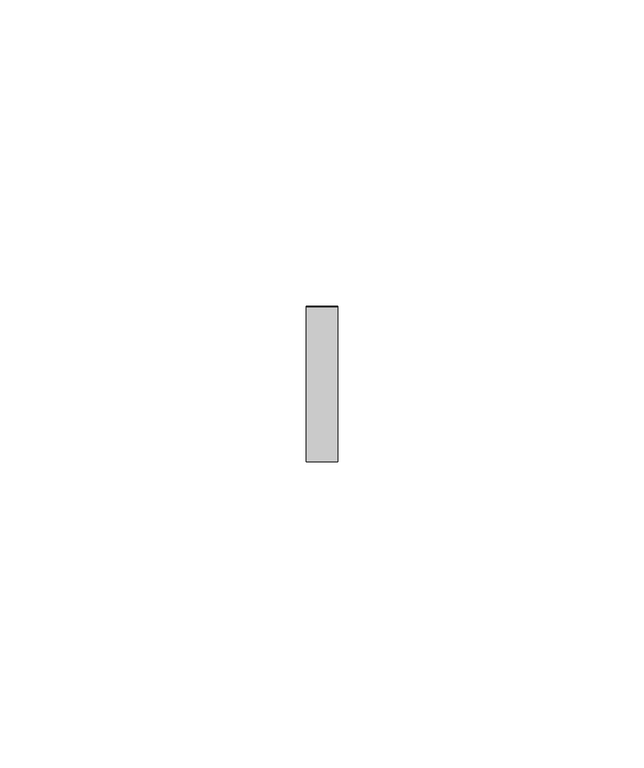
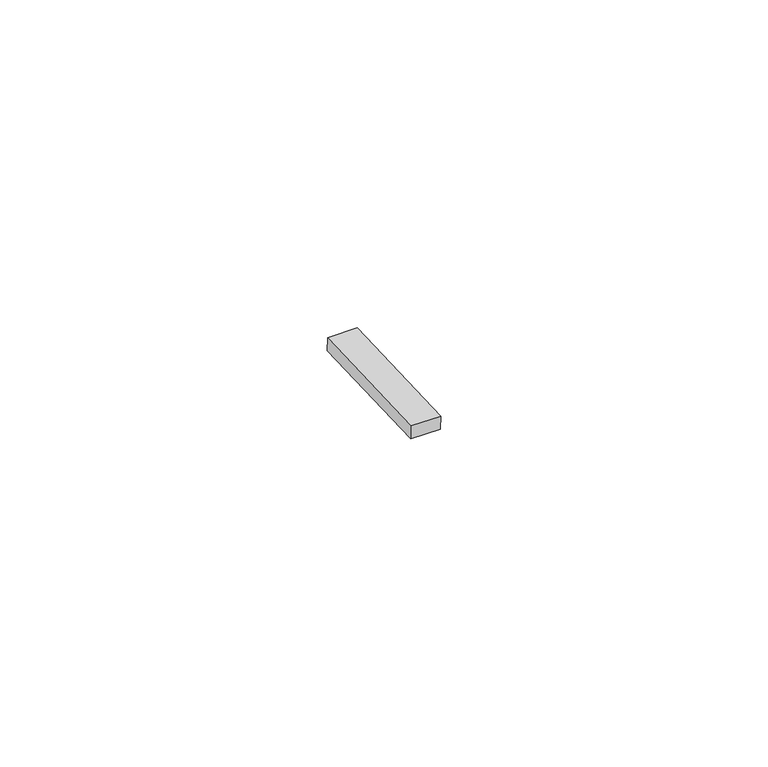
"""IFC4 building model written with IfcOpenShell, lengths in millimetres: proxy geometry, Inner panel:Inner panel:1:Inner panel:1 : Inner panel:Inner panel:300324:2:Inner panel:1:Inner panel:1 : Inner panel:Inner panel:300324:2 : Inner panel:Inner panel:1:Inner panel:1 : Inner panel:Inner panel:300324:300043:125 : Inner panel:Inner panel:1:Inner panel:1 : Inner panel:Inner panel:300324:2:Inner panel:1:Inner panel:1 : Inner panel:Inner panel:300324:2 : Inner panel:Inner panel:1:Inner panel:1 : Inner panel:Inner panel:300324:300043:308120."""

from ifc_helpers import new_model, si_unit, frame, origin, place, context, project, spatial, polyline, outline, extrude, source, transform, mapped, element, save


def generic_models_ade7059a(model_context):
    return source(origin(), model_context, "Body", "SweptSolid", [
        extrude(outline(polyline([(0.0, -25.4), (0.0, 0.0), (5.2138089, 0.0), (5.2138089, -25.4), (0.0, -25.4)])), frame((591904.595117, -578253.2828061, 3981.0403755), z_axis=(0.0, -0.041630544712223896, 0.9991330730923502), x_axis=(-1.0, 0.0, 0.0)), (0.0, 0.0, 1.0), 2.4763745),
    ])


if __name__ == "__main__":
    model = new_model("IFC4")
    model_context = context("Model", 3, world=origin())
    ifc_project = project(units=[si_unit("LENGTHUNIT", "METRE", prefix="MILLI")], contexts=[model_context])
    site = spatial("IfcSite", under=ifc_project)
    building = spatial("IfcBuilding", under=site)
    placement = place(None, origin())
    generic_models_shape = generic_models_ade7059a(model_context)
    element("IfcBuildingElementProxy", 1, Name="Inner panel:Inner panel:1:Inner panel:1 : Inner panel:Inner panel:300324:2:Inner panel:1:Inner panel:1 : Inner panel:Inner panel:300324:2 : Inner panel:Inner panel:1:Inner panel:1 : Inner panel:Inner panel:300324:300043:125 : Inner panel:Inner panel:1:Inner panel:1 : Inner panel:Inner panel:300324:2:Inner panel:1:Inner panel:1 : Inner panel:Inner panel:300324:2 : Inner panel:Inner panel:1:Inner panel:1 : Inner panel:Inner panel:300324:300043:308120", ObjectType="Inner panel:Inner panel:1:Inner panel:1 : Inner panel:Inner panel:300324:2:Inner panel:1:Inner panel:1 : Inner panel:Inner panel:300324:2 : Inner panel:Inner panel:1:Inner panel:1 : Inner panel:Inner panel:300324:300043:125 : Inner panel:Inner panel:1:Inner panel:1 : Inner panel:Inner panel:300324:2:Inner panel:1:Inner panel:1 : Inner panel:Inner panel:300324:2 : Inner panel:Inner panel:1:Inner panel:1 : Inner panel:Inner panel:300324:300043:308120", at=placement, inside=building, context=model_context, shape_type="MappedRepresentation", body=[
        mapped(generic_models_shape, transform((0.0, 0.0, 0.0), x_axis=(1.0, 0.0, 0.0), y_axis=(0.0, 1.0, 0.0), z_axis=(0.0, 0.0, 1.0))),
    ])
    save(model, "model.ifc")

# Revit data of these elements
# Type "Inner panel:Inner panel:1:Inner panel:1 : Inner panel:Inner panel:300324:2:Inner panel:1:Inner panel:1 : Inner panel:Inner panel:300324:2 : Inner panel:Inner panel:1:Inner panel:1 : Inner panel:Inner panel:300324:300043:125 : Inner panel:Inner panel:1:Inner panel:1 : Inner panel:Inner panel:300324:2:Inner panel:1:Inner panel:1 : Inner panel:Inner panel:300324:2 : Inner panel:Inner panel:1:Inner panel:1 : Inner panel:Inner panel:300324:300043:308120"
#   NameOverride = "Inner panel:Inner panel:1:Inner panel:1 : Inner panel:Inner panel:300324:2:Inner panel:1:Inner panel:1 : Inner panel:Inner panel:300324:2 : Inner panel:Inner panel:1:Inner panel:1 : Inner panel:Inner panel:300324:300043:308120"
#   ObjectTypeOverride = "Inner panel:1:Inner panel:1 : Inner panel:Inner panel:300324:2 : Inner panel:Inner panel:1:Inner panel:1 : Inner panel:Inner panel:300324:300043"
#   Reference = "Inner panel"
#   Tag = "308120"
# Element 1 (IfcBuildingElementProxy, "Inner panel:Inner panel:1:Inner panel:1 : Inner panel:Inner panel:300324:2:Inner panel:1:Inner panel:1 : Inner panel:Inner panel:300324:2 : Inner panel:Inner panel:1:Inner panel:1 : Inner panel:Inner panel:300324:300043:125 : Inner panel:Inner panel:1:Inner panel:1 : Inner panel:Inner panel:300324:2:Inner panel:1:Inner panel:1 : Inner panel:Inner panel:300324:2 : Inner panel:Inner panel:1:Inner panel:1 : Inner panel:Inner panel:300324:300043:308120")
#   Materials on its faces: "AT CLIP - 1\" WIDE NON ABSORBENT, WEATHER-RESISTANT NEOPRENE/EPDM/SBR FOAM"
# Materials
#   "AT CLIP - 1\" WIDE NON ABSORBENT, WEATHER-RESISTANT NEOPRENE/EPDM/SBR FOAM": class "Generic", colour RGB 85 85 85, transparency 0, Cost = 0
